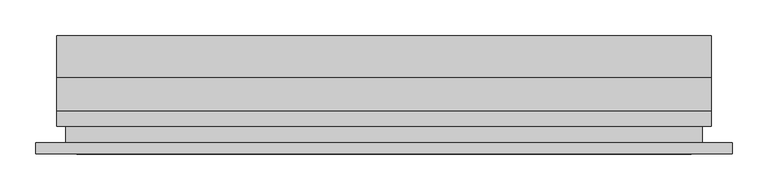
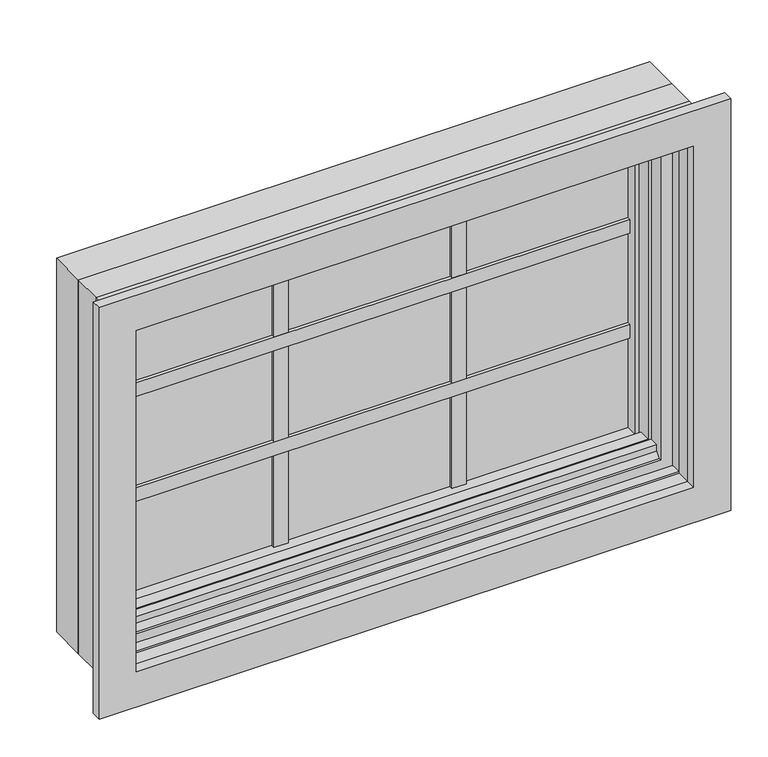
"""IFC4 building model written with IfcOpenShell, lengths in millimetres: proxy geometry, Window-Awning-Andersen-400_Series_Single : Window-Awning-Andersen-400_Series_Single."""

from ifc_helpers import new_model, si_unit, frame, origin, place, context, project, spatial, polyline, outline, extrude, faceted_brep, source, transform, mapped, element, save


def generic_models_9b0c234f(model_context):
    return source(origin(), model_context, "Body", "SolidModel", [
        extrude(outline(polyline([(-400.48815, 12.0054687), (400.4056, 12.0054687), (400.4056, 6.6476562), (-400.48815, 6.6476562), (-400.48815, 12.0054687)])), frame((0.0, 0.0, 1857.3904446), z_axis=(0.0, 0.0, 1.0), x_axis=(1.0, 0.0, 0.0)), (0.0, 0.0, 1.0), 22.225),
        extrude(outline(polyline([(-400.48815, 24.7054687), (400.4056, 24.7054687), (400.4056, 15.1804687), (-400.48815, 15.1804687), (-400.48815, 24.7054687)])), frame((0.0, 0.0, 1857.3904446), z_axis=(0.0, 0.0, 1.0), x_axis=(1.0, 0.0, 0.0)), (0.0, 0.0, 1.0), 22.225),
        extrude(outline(polyline([(-400.48815, 33.2382812), (400.4056, 33.2382812), (400.4056, 27.8804687), (-400.48815, 27.8804687), (-400.48815, 33.2382812)])), frame((0.0, 0.0, 1857.3904446), z_axis=(0.0, 0.0, 1.0), x_axis=(1.0, 0.0, 0.0)), (0.0, 0.0, 1.0), 22.225),
        extrude(outline(polyline([(-400.48815, 12.0054687), (400.4056, 12.0054687), (400.4056, 6.6476562), (-400.48815, 6.6476562), (-400.48815, 12.0054687)])), frame((0.0, 0.0, 1685.9404446), z_axis=(0.0, 0.0, 1.0), x_axis=(1.0, 0.0, 0.0)), (0.0, 0.0, 1.0), 22.225),
        extrude(outline(polyline([(-400.48815, 24.7054687), (400.4056, 24.7054687), (400.4056, 15.1804687), (-400.48815, 15.1804687), (-400.48815, 24.7054687)])), frame((0.0, 0.0, 1685.9404446), z_axis=(0.0, 0.0, 1.0), x_axis=(1.0, 0.0, 0.0)), (0.0, 0.0, 1.0), 22.225),
        extrude(outline(polyline([(-400.48815, 33.2382812), (400.4056, 33.2382812), (400.4056, 27.8804687), (-400.48815, 27.8804687), (-400.48815, 33.2382812)])), frame((0.0, 0.0, 1685.9404446), z_axis=(0.0, 0.0, 1.0), x_axis=(1.0, 0.0, 0.0)), (0.0, 0.0, 1.0), 22.225),
        extrude(outline(polyline([(-148.3402333, 12.0054687), (-126.1152333, 12.0054687), (-126.1152333, 6.6476562), (-148.3402333, 6.6476562), (-148.3402333, 12.0054687)])), frame((0.0, 0.0, 1536.7154446), z_axis=(0.0, 0.0, 1.0), x_axis=(1.0, 0.0, 0.0)), (0.0, 0.0, 1.0), 492.125),
        extrude(outline(polyline([(-148.3402333, 24.7054687), (-126.1152333, 24.7054687), (-126.1152333, 15.1804687), (-148.3402333, 15.1804687), (-148.3402333, 24.7054687)])), frame((0.0, 0.0, 1536.7154446), z_axis=(0.0, 0.0, 1.0), x_axis=(1.0, 0.0, 0.0)), (0.0, 0.0, 1.0), 492.125),
        extrude(outline(polyline([(-148.3402333, 33.2382812), (-126.1152333, 33.2382812), (-126.1152333, 27.8804687), (-148.3402333, 27.8804687), (-148.3402333, 33.2382812)])), frame((0.0, 0.0, 1536.7154446), z_axis=(0.0, 0.0, 1.0), x_axis=(1.0, 0.0, 0.0)), (0.0, 0.0, 1.0), 492.125),
        extrude(outline(polyline([(126.0326833, 12.0054687), (148.2576833, 12.0054687), (148.2576833, 6.6476562), (126.0326833, 6.6476562), (126.0326833, 12.0054687)])), frame((0.0, 0.0, 1536.7154446), z_axis=(0.0, 0.0, 1.0), x_axis=(1.0, 0.0, 0.0)), (0.0, 0.0, 1.0), 492.125),
        extrude(outline(polyline([(126.0326833, 24.7054687), (148.2576833, 24.7054687), (148.2576833, 15.1804687), (126.0326833, 15.1804687), (126.0326833, 24.7054687)])), frame((0.0, 0.0, 1536.7154446), z_axis=(0.0, 0.0, 1.0), x_axis=(1.0, 0.0, 0.0)), (0.0, 0.0, 1.0), 492.125),
        extrude(outline(polyline([(126.0326833, 33.2382812), (148.2576833, 33.2382812), (148.2576833, 27.8804687), (126.0326833, 27.8804687), (126.0326833, 33.2382812)])), frame((0.0, 0.0, 1536.7154446), z_axis=(0.0, 0.0, 1.0), x_axis=(1.0, 0.0, 0.0)), (0.0, 0.0, 1.0), 492.125),
        extrude(outline(polyline([(2074.8779446, -444.93815), (1493.8529446, -444.93815), (1493.8529446, 444.8556), (2074.8779446, 444.8556), (2074.8779446, -444.93815)]), holes=[polyline([(2028.8404446, -400.48815), (2028.8404446, 400.4056), (1536.7154446, 400.4056), (1536.7154446, -400.48815), (2028.8404446, -400.48815)])]), frame((0.0, -6.35, 0.0), z_axis=(0.0, 1.0, 0.0), x_axis=(0.0, 0.0, 1.0)), (0.0, 0.0, 1.0), 50.8),
        extrude(outline(polyline([(-400.48815, 27.8804687), (400.4056, 27.8804687), (400.4056, 12.0054687), (-400.48815, 12.0054687), (-400.48815, 27.8804687)])), frame((0.0, 0.0, 1536.7154446), z_axis=(0.0, 0.0, 1.0), x_axis=(1.0, 0.0, 0.0)), (0.0, 0.0, 1.0), 492.125),
        faceted_brep([(-429.0314, -6.35, 2060.956), (-429.0314, -57.15, 2060.956), (429.0314, -57.15, 2060.956), (429.0314, -6.35, 2060.956), (-429.0314, -6.35, 1504.569), (429.0314, -6.35, 1504.569), (429.0314, -53.2892, 1504.569), (-429.0314, -53.2892, 1504.569), (-429.0314, -53.2892, 1507.33125), (-429.0314, -57.15, 1507.33125), (429.0314, -57.15, 1507.33125), (411.1752, -57.15, 1522.0188), (-411.1752, -57.15, 1522.0188), (-411.1752, -57.15, 2040.763), (411.1752, -57.15, 2040.763), (-411.1752, -46.175563, 1541.0942), (-411.1752, -31.75, 1541.0942), (-411.1752, -31.75, 2040.763), (-411.1752, -53.3654, 1522.0188), (-411.1752, -46.175563, 1530.6587599), (411.1752, -31.75, 1541.0942), (411.1752, -31.75, 2040.763), (406.4, -31.75, 1543.05), (-406.4, -31.75, 1543.05), (-406.4, -31.75, 2031.603125), (406.4, -31.75, 2031.603125), (-406.4, -13.1318, 1543.05), (-406.4, -6.35, 1535.938), (-406.4, -6.35, 2031.603125), (406.4, -6.35, 1535.938), (406.4, -6.35, 2031.603125), (406.4, -13.1318, 1543.05), (411.1752, -46.175563, 1541.0942), (411.1752, -46.175563, 1530.6587599), (411.1752, -53.3654, 1522.0188), (429.0314, -53.2892, 1507.33125), (-429.41875, -73.9267, 2061.36875), (-429.41875, -53.2892, 2061.36875), (429.41875, -53.2892, 2061.36875), (429.41875, -73.9267, 2061.36875), (-457.2, -53.2892, 2089.15), (-457.2, -73.9267, 2089.15), (457.2, -73.9267, 2089.15), (457.2, -53.2892, 2089.15), (429.41875, -53.2892, 1507.33125), (429.41875, -73.9267, 1507.33125), (457.2, -73.9267, 1479.55), (457.2, -53.2892, 1479.55), (-429.41875, -53.2892, 1507.33125), (-429.41875, -73.9267, 1507.33125), (-457.2, -73.9267, 1479.55), (-457.2, -53.2892, 1479.55)], [[[0, 1, 2, 3]], [[4, 5, 6, 7]], [[1, 0, 4, 7, 8, 9]], [[2, 1, 9, 10], [11, 12, 13, 14]], [[15, 16, 17, 13, 12, 18, 19]], [[16, 20, 21, 17], [22, 23, 24, 25]], [[23, 26, 27, 28, 24]], [[5, 4, 0, 3], [27, 29, 30, 28]], [[31, 22, 25, 30, 29]], [[20, 32, 33, 34, 11, 14, 21]], [[3, 2, 10, 35, 6, 5]], [[23, 22, 31, 26]], [[29, 27, 26, 31]], [[15, 32, 20, 16]], [[32, 15, 19, 33]], [[33, 19, 18, 34]], [[12, 11, 34, 18]], [[14, 13, 17, 21]], [[25, 24, 28, 30]], [[36, 37, 38, 39]], [[40, 41, 42, 43]], [[39, 38, 44, 45]], [[43, 42, 46, 47]], [[45, 44, 35, 10, 9, 8, 48, 49]], [[47, 46, 50, 51]], [[37, 36, 49, 48]], [[42, 41, 50, 46], [36, 39, 45, 49]], [[41, 40, 51, 50]], [[40, 43, 47, 51], [38, 37, 48, 8, 7, 6, 35, 44]]]),
        extrude(outline(polyline([(2089.15, -457.2), (1479.55, -457.2), (1479.55, 457.2), (2089.15, 457.2), (2089.15, -457.2)]), holes=[polyline([(2060.956, -429.0314), (2060.956, 429.0314), (1504.569, 429.0314), (1504.569, -429.0314), (2060.956, -429.0314)])]), frame((0.0, -53.2892, 0.0), z_axis=(0.0, 1.0, 0.0), x_axis=(0.0, 0.0, 1.0)), (0.0, 0.0, 1.0), 46.9392),
        extrude(outline(polyline([(2089.15, -457.2), (1479.55, -457.2), (1479.55, 457.2), (2089.15, 457.2), (2089.15, -457.2)]), holes=[polyline([(2074.8470554, -444.8556), (2074.8470554, 444.8556), (1493.8529446, 444.8556), (1493.8529446, -444.8556), (2074.8470554, -444.8556)])]), frame((0.0, -6.35, 0.0), z_axis=(0.0, 1.0, 0.0), x_axis=(0.0, 0.0, 1.0)), (0.0, 0.0, 1.0), 58.7248),
        extrude(outline(polyline([(2118.51875, 486.56875), (2118.51875, -486.56875), (1447.419, -486.56875), (1447.419, 486.56875), (2118.51875, 486.56875)]), holes=[polyline([(2061.36875, 429.41875), (1504.569, 429.41875), (1504.569, -429.41875), (2061.36875, -429.41875), (2061.36875, 429.41875)])]), frame((0.0, -112.7125, 0.0), z_axis=(0.0, 1.0, 0.0), x_axis=(0.0, 0.0, 1.0)), (0.0, 0.0, 1.0), 15.875),
        extrude(outline(polyline([(2076.45, 444.5), (2076.45, -444.5), (1492.25, -444.5), (1492.25, 444.5), (2076.45, 444.5)]), holes=[polyline([(2061.36875, 429.41875), (1504.569, 429.41875), (1504.569, -429.41875), (2061.36875, -429.41875), (2061.36875, 429.41875)])]), frame((0.0, -96.8375, 0.0), z_axis=(0.0, 1.0, 0.0), x_axis=(0.0, 0.0, 1.0)), (0.0, 0.0, 1.0), 43.65625),
    ])


if __name__ == "__main__":
    model = new_model("IFC4")
    model_context = context("Model", 3, world=origin())
    ifc_project = project(units=[si_unit("LENGTHUNIT", "METRE", prefix="MILLI")], contexts=[model_context])
    site = spatial("IfcSite", under=ifc_project)
    building = spatial("IfcBuilding", under=site)
    placement = place(None, origin())
    generic_models_shape = generic_models_9b0c234f(model_context)
    element("IfcBuildingElementProxy", 1, Name="Window-Awning-Andersen-400_Series_Single : Window-Awning-Andersen-400_Series_Single", ObjectType="Window-Awning-Andersen-400_Series_Single : Window-Awning-Andersen-400_Series_Single", at=placement, inside=building, context=model_context, shape_type="MappedRepresentation", body=[
        mapped(generic_models_shape, transform((0.0, 0.0, 0.0), x_axis=(1.0, 0.0, 0.0), y_axis=(0.0, 1.0, 0.0), z_axis=(0.0, 0.0, 1.0))),
    ])
    save(model, "model.ifc")

# Revit data of these elements
# Type "Window-Awning-Andersen-400_Series_Single : Window-Awning-Andersen-400_Series_Single"
#   Learn About These Parameters = "http://www.andersenwindows.com/for-professionals/cad-symbols-bim-support-window-doors/bim-support"
#   ..Jamb Condition Number 1 = "Extension Jamb Only"
#   ..Jamb Condition Number 2 = "Narrow Drywall Return"
#   ..Jamb Condition Number 3 = "Wide Drywall Return"
#   Available Grille Bar Sizes = "3/4'', 7/8'', 1 1/8'', 2 1/4''"
#   Between Glass Grille Bar Sizes = "3/4'', 1''"
#   ..Pattern Number 1 = "Colonial"
#   ..Pattern Number 2 = "Modified Colonial"
#   ..Pattern Number 3 = "Prairie"
#   ..Pattern Number 4 = "Short Fractional"
#   ..Pattern Number 5 = "Tall Fractional"
#   ..Exterior Trim Number 0 = "No Exterior Trim"
#   ..Exterior Trim Number 1 = "Brick Mould"
#   ..Exterior Trim Number 2 = "3 1/2'' Flat Casing"
#   ..Exterior Trim Number 3 = "4 1/2'' Flat Casing"
#   URL = "www.andersenwindows.com"
#   Type Comments = "Vinyl-clad wood awning window"
#   Product Documentation Link = "https://www.andersenwindows.com/windows-and-doors/windows/awning-windows/400-series-awning-window/"
#   Model = "400-Series Awning"
#   Manufacturer = "Andersen Corporation"
#   Family Version = "01.01.19"
#   Designation = "CMT"
#   Description = "Vinyl-clad wood awning window"
#   Assembly Code = "B2020100"
#   XPanelWidth = 2' - 11 1/32"
#   XPanelHeight = 1' - 10 7/8"
#   Width = 3' - 0"
#   Visual Light Transmittance = 0.48
#   Thermal Resistance (R) = 0.628713 (stored number, unit not read)
#   Solar Heat Gain Coefficient = 0.21
#   Rough Width = 3' - 0 1/2"
#   Rough Height = 2' - 0 1/2"
#   Height = 2' - 0"
#   Heat Transfer Coefficient (U) = 1.58991 (stored number, unit not read)
#   Grille Bar Size = 0' - 0 7/8"
#   xjamb S1 [instance default] = 0' - 1 23/32"
#   sill nose1 = 0' - 1 13/16"
#   sill nose 2 = 0' - 1 15/16"
#   casingS2 = 0' - 0 3/16"
#   casingS1 = 0' - 0 3/16"
#   casing4 = 0' - 4 1/4"
#   casing3 = 0' - 0 1/2"
#   casing2 = 0' - 0 7/8"
#   casing1 = 0' - 0 1/4"
#   Xjamb 2 = 0' - 0 1/2"
#   Xjamb 1 = 0' - 1 3/32"
#   Wall Thickness [instance default] = 0' - 6"
#   Wall Depth [instance default] = 0' - 4 9/16"
#   Void Offset 2 = 0' - 0"
#   Void Offset 1 = 0' - 0"
#   Void Depth [instance default] = 0' - 2 7/16"
#   VGB DLO = 0' - 9.91667"
#   TS V DLO = 1' - 7 3/8"
#   TS V Bar Length = 1' - 7 3/8"
#   TS SH DLO = 1' - 0 1/16"
#   TS HGB DLO = 0' - 5 7/8"
#   Step Jamb2 = 0' - 0 13/16"
#   Step Jamb1 = 0' - 1 1/8"
#   Sill Stop Dim [instance default] = 0' - 2 1/2"
#   SGO = 0' - 2 1/4"
#   Rough Opening Offset = 0' - 0 1/4"
#   Plan Exterior Mask 2 [instance default] = 0' - 1 3/8"
#   Plan Exterior Mask [instance default] = 0' - 1 1/16"
#   Masonry Width = 3' - 0 1/2"
#   Masonry Opening Offset = 0' - 0 1/4"
#   Masonry Height = 2' - 0 1/2"
#   JGO = 0' - 2 1/4"
#   Interior Casing Size = 0' - 2 1/4"
#   Horizontal Craftsman Bar Size = 0' - 0 7/8"
#   Head Stop Dim [instance default] = 0' - 2 17/64"
#   HGO = 0' - 2 3/8"
#   H DLO = 2' - 7 1/2"
#   Default Sill Height = 4' - 10"
#   Coarse Plan [instance default] = 0' - 4 9/16"
#   TFL = 2
#   TFB = 1
#   LWide = 3
#   Handing Visibility = yes
#   Fractional Lights Wide = 3
#   Fractional Lights High = 5
#   Enter Jamb Condition = 1
#   Interior Casing = yes
#   Enter Pattern Number = 1
#   . . Lights Wide = 3
#   . . Lights High = 3
#   Extension Jamb = yes
#   Enter Exterior Trim Number = 0
#   Interior Grille Bar = yes
#   Exterior Grille Bar = yes
#   Between Glass Grille Bar = yes
#   xjamb Visibility [instance default] = yes
#   VeriLock Sensor [instance default] = no
#   V Bars = 2
#   TS S V = no
#   TS S H Craftsman = no
#   TS S H = no
#   TS M V = yes
#   TS M H = yes
#   TS H Bars = 2
#   Step Visibility = no
#   Push Out Stop Visibility [instance default] = no
#   Plan Exterior Mask Visibility [instance default] = yes
#   Nail Fin Visibility = yes
#   Interior Trim Visibility = yes
#   Crank Out Stop Visibility [instance default] = yes
#   Casing Visibility = no
#   Bar Center Line = 2
#   Glazing Material = DOUBLE HUNG WINDOWS
#   Exterior Unit Finish = Vinyl - Andersen - White
#   Interior Material = Wood - Andersen - Pine
#   Exterior Trim Finish = Fibrex Composite - Andersen - White
#   Between Glass Grille Bar Finish = Stainless Steel - Andersen - Standard
#   Wall Closure = (empty or 0)
# Element 1 (IfcBuildingElementProxy, "Window-Awning-Andersen-400_Series_Single : Window-Awning-Andersen-400_Series_Single")
#   Wall Thickness = 0' - 7 5/8"
#   Void Depth = 0' - 4 1/16"
#   Plan Exterior Mask 2 = 0' - 3"
#   Materials on its faces: "Wood - Andersen - Pine", "Vinyl - Andersen - White", "Stainless Steel - Andersen - Standard", "DOUBLE HUNG WINDOWS"
# Materials
#   "DOUBLE HUNG WINDOWS": class "Glass", colour RGB 236 240 239, transparency 0.85, Cost = 0
#   "Vinyl - Andersen - White": class "Plastic", colour RGB 241 238 228, transparency 0, Description = "White vinyl finish", Cost = 0
#   "Wood - Andersen - Pine": class "Wood", colour RGB 235 199 148, transparency 0, Description = "Pinus Echinata", Cost = 0
#   "Fibrex Composite - Andersen - White": class "Plastic", colour RGB 241 238 228, transparency 0, Manufacturer = "Andersen", Description = "Wood fiber and thermoplastic polymer composite material", Cost = 0
#   "Stainless Steel - Andersen - Standard": class "Metal", colour RGB 149 149 150, transparency 0, Cost = 0
